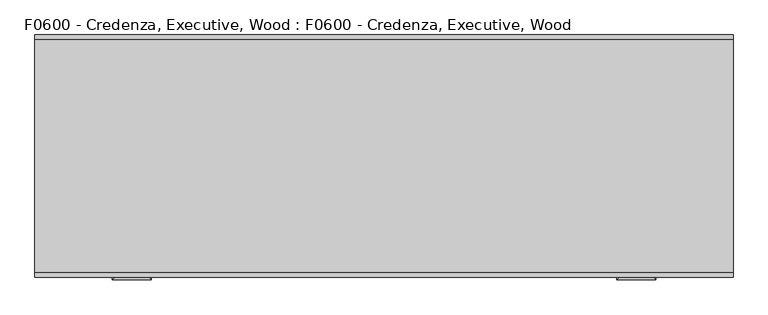
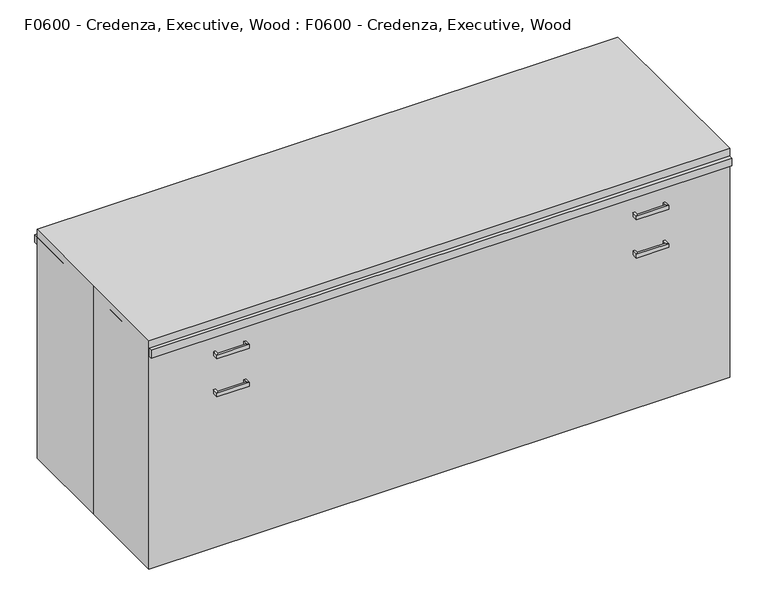
"""IFC4 building model written with IfcOpenShell, lengths in millimetres: proxy geometry, F0600 - Credenza, Executive, Wood : F0600 - Credenza, Executive, Wood."""

import ifcopenshell
import ifcopenshell.guid

model = None  # the IFC model being written
_history = None  # IfcOwnerHistory: only IFC2X3 demands one
_inside = {}  # id of a spatial element -> (the spatial element, [elements in it])
_under = {}  # id of a project, library or spatial element -> (it, [spatial elements below it])
_declared = {}  # id of a project -> (the project, [libraries it declares])
_typed = {}  # id of a type object -> (the type object, [elements of that type])
_made_of = {}  # id of a material, layer set ... -> (it, [elements and type objects made of it])


def new_model(schema):
    """Start an empty IFC model of exactly this schema.

    Asked for "IFC4X3", IfcOpenShell would pick the latest addendum, in which some entities
    have other attributes; the version numbers below select the first issue.
    IFC2X3 requires an IfcOwnerHistory on every rooted entity: one is made here for all.
    """
    global model, _history
    if schema == "IFC4X3":
        model = ifcopenshell.file(schema_version=(4, 3, 0, 0))
    else:
        model = ifcopenshell.file(schema=schema)
    _inside.clear()
    _under.clear()
    _declared.clear()
    _typed.clear()
    _made_of.clear()
    _history = None
    if model.schema == "IFC2X3":
        org = make("IfcOrganization", Name="unknown")
        user = make(
            "IfcPersonAndOrganization",
            ThePerson=make("IfcPerson", FamilyName="unknown"),
            TheOrganization=org,
        )
        app = make(
            "IfcApplication",
            ApplicationDeveloper=org,
            Version="unknown",
            ApplicationFullName="unknown",
            ApplicationIdentifier="unknown",
        )
        _history = make(
            "IfcOwnerHistory",
            OwningUser=user,
            OwningApplication=app,
            ChangeAction="ADDED",
            CreationDate=0,
        )
    return model


def make(cls, **values):
    """One entity of the class cls with the attributes given. An attribute that is None is left unset."""
    return model.create_entity(
        cls, **{name: value for name, value in values.items() if value is not None}
    )


def rooted(cls, **values):
    """An entity with a GlobalId (a new one), such as an element, a storey or a relation."""
    return make(cls, GlobalId=ifcopenshell.guid.new(), OwnerHistory=_history, **values)


def si_unit(unit_type, name, prefix=None):
    """IfcSIUnit, for example si_unit("LENGTHUNIT", "METRE", prefix="MILLI")."""
    return make("IfcSIUnit", UnitType=unit_type, Prefix=prefix, Name=name)


def assignment(units):
    """IfcUnitAssignment: the units of a project."""
    return None if units is None else make("IfcUnitAssignment", Units=units)


def point(xyz):
    """IfcCartesianPoint."""
    return None if xyz is None else make("IfcCartesianPoint", Coordinates=xyz)


def direction(xyz):
    """IfcDirection."""
    return None if xyz is None else make("IfcDirection", DirectionRatios=xyz)


def frame(location, z_axis=None, x_axis=None):
    """IfcAxis2Placement3D, a coordinate frame: its origin and axes. An axis left out is left unset."""
    return make(
        "IfcAxis2Placement3D",
        Location=point(location),
        Axis=direction(z_axis),
        RefDirection=direction(x_axis),
    )


def origin():
    """The frame at (0, 0, 0) with its axes left unset."""
    return frame((0.0, 0.0, 0.0))


def origin_with_axes():
    """The frame at (0, 0, 0) with the z axis (0, 0, 1) and the x axis (1, 0, 0) written out."""
    return frame((0.0, 0.0, 0.0), z_axis=(0.0, 0.0, 1.0), x_axis=(1.0, 0.0, 0.0))


def place(relative_to, where):
    """IfcLocalPlacement: puts the frame where relative to a parent placement (None: the world)."""
    return make(
        "IfcLocalPlacement", PlacementRelTo=relative_to, RelativePlacement=where
    )


def context(
    kind, dimensions, precision=None, world=None, true_north=None, identifier=None
):
    """IfcGeometricRepresentationContext, for example the 3D "Model" context."""
    return make(
        "IfcGeometricRepresentationContext",
        ContextIdentifier=identifier,
        ContextType=kind,
        CoordinateSpaceDimension=dimensions,
        Precision=precision,
        WorldCoordinateSystem=world,
        TrueNorth=true_north,
    )


def project(units=None, contexts=None):
    """IfcProject with its units and contexts."""
    return rooted(
        "IfcProject",
        Name="project",
        RepresentationContexts=contexts,
        UnitsInContext=assignment(units),
    )


def spatial(cls, under=None, at=None, **own):
    """A site, building, storey or space (cls), placed at a placement, below another one or the project."""
    s = rooted(cls, ObjectPlacement=at, **own)
    if under is not None:
        _under.setdefault(under.id(), (under, []))[1].append(s)
    return s


def polyline(points):
    """IfcPolyline through the points."""
    return make("IfcPolyline", Points=[point(p) for p in points])


def outline(outer, holes=None, kind="AREA"):
    """IfcArbitraryClosedProfileDef: a profile drawn as a closed curve; with holes, ...WithVoids."""
    if holes is None:
        return make("IfcArbitraryClosedProfileDef", ProfileType=kind, OuterCurve=outer)
    return make(
        "IfcArbitraryProfileDefWithVoids",
        ProfileType=kind,
        OuterCurve=outer,
        InnerCurves=holes,
    )


def extrude(swept, where, along, depth):
    """IfcExtrudedAreaSolid: the profile swept, set in the frame where, extruded along a direction by depth."""
    return make(
        "IfcExtrudedAreaSolid",
        SweptArea=swept,
        Position=where,
        ExtrudedDirection=direction(along),
        Depth=depth,
    )


def faces_of(points, faces, orient=None, outer=None):
    """IfcFace entities. A face is a list of loops; a loop is a list of indices into points, from 0.

    orient and outer hold one flag for each loop. By default every Orientation is true, the
    first loop of a face is its IfcFaceOuterBound and the others are IfcFaceBound.
    """
    made = []
    for i, loops in enumerate(faces):
        bounds = []
        for j, loop in enumerate(loops):
            is_outer = j == 0 if outer is None else outer[i][j]
            bounds.append(
                make(
                    "IfcFaceOuterBound" if is_outer else "IfcFaceBound",
                    Bound=make("IfcPolyLoop", Polygon=[points[k] for k in loop]),
                    Orientation=True if orient is None else orient[i][j],
                )
            )
        made.append(make("IfcFace", Bounds=bounds))
    return made


def faceted_brep(points, faces, orient=None, outer=None, voids=None):
    """IfcFacetedBrep: a solid bounded by flat faces; with voids (closed shells), ...WithVoids."""
    shared = [point(p) for p in points]
    hull = make("IfcClosedShell", CfsFaces=faces_of(shared, faces, orient, outer))
    if voids is None:
        return make("IfcFacetedBrep", Outer=hull)
    return make(
        "IfcFacetedBrepWithVoids",
        Outer=hull,
        Voids=[
            make(cls, CfsFaces=faces_of(shared, fs, o, b)) for cls, fs, o, b in voids
        ],
    )


def shape(context_of_items, identifier, shape_type, items):
    """IfcShapeRepresentation: the items that make up one representation, for example the "Body"."""
    return make(
        "IfcShapeRepresentation",
        ContextOfItems=context_of_items,
        RepresentationIdentifier=identifier,
        RepresentationType=shape_type,
        Items=items,
    )


def source(mapping_origin, context_of_items, identifier, shape_type, items):
    """IfcRepresentationMap: a shape defined once, which mapped items show again and again."""
    return make(
        "IfcRepresentationMap",
        MappingOrigin=mapping_origin,
        MappedRepresentation=shape(context_of_items, identifier, shape_type, items),
    )


def transform(
    local_origin,
    x_axis=None,
    y_axis=None,
    z_axis=None,
    scale=None,
    scale2=None,
    scale3=None,
    uniform=True,
):
    """IfcCartesianTransformationOperator3D, or its non-uniform kind. x_axis, y_axis, z_axis: its Axis1, 2, 3."""
    if uniform:
        return make(
            "IfcCartesianTransformationOperator3D",
            Axis1=direction(x_axis),
            Axis2=direction(y_axis),
            LocalOrigin=point(local_origin),
            Scale=scale,
            Axis3=direction(z_axis),
        )
    return make(
        "IfcCartesianTransformationOperator3DnonUniform",
        Axis1=direction(x_axis),
        Axis2=direction(y_axis),
        LocalOrigin=point(local_origin),
        Scale=scale,
        Axis3=direction(z_axis),
        Scale2=scale2,
        Scale3=scale3,
    )


def mapped(mapping_source, mapping_target):
    """IfcMappedItem: shows the shape of a source again, moved by a transform."""
    return make(
        "IfcMappedItem", MappingSource=mapping_source, MappingTarget=mapping_target
    )


def made_of(thing, what):
    """Note that an element or type object is made of a material, layer set ...; save() writes the relation."""
    if what is not None:
        _made_of.setdefault(what.id(), (what, []))[1].append(thing)
    return thing


def element(
    cls,
    number,
    at=None,
    inside=None,
    cuts=None,
    type_object=None,
    material=None,
    context=None,
    identifier="Body",
    shape_type=None,
    held_by="IfcProductDefinitionShape",
    body=None,
    shapes=None,
    **own,
):
    """One element of the class cls, such as IfcWall. Its Tag is "e" and its number.

    at: its placement. inside: the storey or other place that contains it. cuts: it is an
    opening in that element (IfcRelVoidsElement). A single representation is given by context,
    identifier, shape_type and body (its items); several are given by shapes. held_by: the class
    of the entity that holds the representations. save() writes the other relations.
    """
    e = rooted(cls, Tag="e%d" % number, ObjectPlacement=at, **own)
    if body is not None:
        shapes = [shape(context, identifier, shape_type, body)]
    if shapes is not None:
        e.Representation = make(held_by, Representations=shapes)
    if inside is not None:
        _inside.setdefault(inside.id(), (inside, []))[1].append(e)
    if cuts is not None:
        rooted(
            "IfcRelVoidsElement", RelatingBuildingElement=cuts, RelatedOpeningElement=e
        )
    if type_object is not None:
        _typed.setdefault(type_object.id(), (type_object, []))[1].append(e)
    return made_of(e, material)


def aggregate(whole, parts):
    """IfcRelAggregates: a whole, such as a stair, and the parts it consists of."""
    return rooted("IfcRelAggregates", RelatingObject=whole, RelatedObjects=parts)


def save(model, path):
    """Write the relations noted so far, then the file.

    IfcRelAggregates (storeys below a building ...), IfcRelContainedInSpatialStructure (elements
    in a storey), IfcRelDefinesByType, IfcRelAssociatesMaterial and IfcRelDeclares: one each for
    every whole, place, type object, material and project.
    """
    for whole, parts in _under.values():
        aggregate(whole, parts)
    for where, things in _inside.values():
        rooted(
            "IfcRelContainedInSpatialStructure",
            RelatedElements=things,
            RelatingStructure=where,
        )
    for kind, things in _typed.values():
        rooted("IfcRelDefinesByType", RelatedObjects=things, RelatingType=kind)
    for what, things in _made_of.values():
        rooted("IfcRelAssociatesMaterial", RelatedObjects=things, RelatingMaterial=what)
    for by, libraries in _declared.values():
        rooted("IfcRelDeclares", RelatingContext=by, RelatedDefinitions=libraries)
    model.write(path)


def f0600_credenza_executive_wood_f0600_credenza_executive_wood_160093f6(model_context):
    return source(origin(), model_context, "Body", "SolidModel", [
        faceted_brep([(-704.85, -298.45, 527.05), (-704.85, -298.45, 514.35), (-711.2, -298.45, 514.35), (-711.2, -298.45, 527.05), (-704.85, -317.5, 527.05), (-704.85, -317.5, 514.35), (-711.2, -323.85, 514.35), (-711.2, -323.85, 527.05), (-615.95, -317.5, 527.05), (-615.95, -317.5, 514.35), (-609.6, -323.85, 514.35), (-609.6, -323.85, 527.05), (-615.95, -298.45, 527.05), (-609.6, -298.45, 527.05), (-609.6, -298.45, 514.35), (-615.95, -298.45, 514.35)], [[[0, 1, 2, 3]], [[1, 0, 4, 5]], [[2, 1, 5, 6]], [[3, 2, 6, 7]], [[0, 3, 7, 4]], [[5, 4, 8, 9]], [[6, 5, 9, 10]], [[7, 6, 10, 11]], [[4, 7, 11, 8]], [[12, 13, 14, 15]], [[9, 8, 12, 15]], [[10, 9, 15, 14]], [[11, 10, 14, 13]], [[8, 11, 13, 12]]]),
        faceted_brep([(-704.85, -298.45, 654.05), (-704.85, -298.45, 641.35), (-711.2, -298.45, 641.35), (-711.2, -298.45, 654.05), (-704.85, -317.5, 654.05), (-704.85, -317.5, 641.35), (-711.2, -323.85, 641.35), (-711.2, -323.85, 654.05), (-615.95, -317.5, 654.05), (-615.95, -317.5, 641.35), (-609.6, -323.85, 641.35), (-609.6, -323.85, 654.05), (-615.95, -298.45, 654.05), (-609.6, -298.45, 654.05), (-609.6, -298.45, 641.35), (-615.95, -298.45, 641.35)], [[[0, 1, 2, 3]], [[1, 0, 4, 5]], [[2, 1, 5, 6]], [[3, 2, 6, 7]], [[0, 3, 7, 4]], [[5, 4, 8, 9]], [[6, 5, 9, 10]], [[7, 6, 10, 11]], [[4, 7, 11, 8]], [[12, 13, 14, 15]], [[9, 8, 12, 15]], [[10, 9, 15, 14]], [[11, 10, 14, 13]], [[8, 11, 13, 12]]]),
        faceted_brep([(615.95, -298.45, 654.1373112), (615.95, -298.45, 641.4373112), (609.6, -298.45, 641.4373112), (609.6, -298.45, 654.1373112), (615.95, -317.5, 654.1373112), (615.95, -317.5, 641.4373112), (609.6, -323.85, 641.4373112), (609.6, -323.85, 654.1373112), (704.85, -317.5, 654.1373112), (704.85, -317.5, 641.4373112), (711.2, -323.85, 641.4373112), (711.2, -323.85, 654.1373112), (704.85, -298.45, 654.1373112), (711.2, -298.45, 654.1373112), (711.2, -298.45, 641.4373112), (704.85, -298.45, 641.4373112)], [[[0, 1, 2, 3]], [[1, 0, 4, 5]], [[2, 1, 5, 6]], [[3, 2, 6, 7]], [[0, 3, 7, 4]], [[5, 4, 8, 9]], [[6, 5, 9, 10]], [[7, 6, 10, 11]], [[4, 7, 11, 8]], [[12, 13, 14, 15]], [[9, 8, 12, 15]], [[10, 9, 15, 14]], [[11, 10, 14, 13]], [[8, 11, 13, 12]]]),
        faceted_brep([(615.95, -298.45, 527.05), (615.95, -298.45, 514.35), (609.6, -298.45, 514.35), (609.6, -298.45, 527.05), (615.95, -317.5, 527.05), (615.95, -317.5, 514.35), (609.6, -323.85, 514.35), (609.6, -323.85, 527.05), (704.85, -317.5, 527.05), (704.85, -317.5, 514.35), (711.2, -323.85, 514.35), (711.2, -323.85, 527.05), (704.85, -298.45, 527.05), (711.2, -298.45, 527.05), (711.2, -298.45, 514.35), (704.85, -298.45, 514.35)], [[[0, 1, 2, 3]], [[1, 0, 4, 5]], [[2, 1, 5, 6]], [[3, 2, 6, 7]], [[0, 3, 7, 4]], [[5, 4, 8, 9]], [[6, 5, 9, 10]], [[7, 6, 10, 11]], [[4, 7, 11, 8]], [[12, 13, 14, 15]], [[9, 8, 12, 15]], [[10, 9, 15, 14]], [[11, 10, 14, 13]], [[8, 11, 13, 12]]]),
        extrude(outline(polyline([(-914.4, 304.8), (914.4, 304.8), (914.4, -304.8), (-914.4, -304.8), (-914.4, 0.0), (-914.4, 304.8)])), origin_with_axes(), (0.0, 0.0, 1.0), 762.0),
        faceted_brep([(889.0, 317.5, 711.2), (-889.0, 317.5, 711.2), (-889.0, -292.1, 711.2), (889.0, -292.1, 711.2), (889.0, 317.5, 152.4), (889.0, -292.1, 152.4), (-889.0, -292.1, 152.4), (-889.0, 317.5, 152.4), (-431.8, -292.1, 692.15), (431.8, -292.1, 692.15), (431.8, -292.1, 171.45), (-431.8, -292.1, 171.45), (431.8, 298.45, 692.15), (-431.8, 298.45, 692.15), (-431.8, 298.45, 171.45), (431.8, 298.45, 171.45)], [[[0, 1, 2, 3]], [[4, 5, 6, 7]], [[1, 0, 4, 7]], [[2, 1, 7, 6]], [[3, 2, 6, 5], [8, 9, 10, 11]], [[0, 3, 5, 4]], [[12, 13, 14, 15]], [[13, 12, 9, 8]], [[14, 13, 8, 11]], [[15, 14, 11, 10]], [[12, 15, 10, 9]]]),
        extrude(outline(polyline([(431.8, -259.1517862), (-19.05, -259.1517862), (-19.05, -246.4517862), (431.8, -246.4517862), (431.8, -259.1517862)])), frame((0.0, 0.0, 171.45), z_axis=(0.0, 0.0, 1.0), x_axis=(1.0, 0.0, 0.0)), (0.0, 0.0, 1.0), 520.7),
        extrude(outline(polyline([(20.4311852, -271.8517862), (-431.8, -271.8517862), (-431.8, -259.1517862), (20.4311852, -259.1517862), (20.4311852, -271.8517862)])), frame((0.0, 0.0, 171.45), z_axis=(0.0, 0.0, 1.0), x_axis=(1.0, 0.0, 0.0)), (0.0, 0.0, 1.0), 520.7),
        faceted_brep([(787.4, 317.5, 152.4), (787.4, 215.9, 152.4), (889.0, 215.9, 152.4), (889.0, 317.5, 152.4), (812.8, 317.5, 0.0), (889.0, 317.5, 0.0), (889.0, 241.3, 0.0), (812.8, 241.3, 0.0)], [[[0, 1, 2, 3]], [[4, 5, 6, 7]], [[4, 7, 1, 0]], [[7, 6, 2, 1]], [[6, 5, 3, 2]], [[5, 4, 0, 3]]]),
        extrude(outline(polyline([(869.95, -298.45), (431.8, -298.45), (431.8, -292.1), (869.95, -292.1), (869.95, -298.45)])), frame((0.0, 0.0, 584.2), z_axis=(0.0, 0.0, 1.0), x_axis=(1.0, 0.0, 0.0)), (0.0, 0.0, 1.0), 107.95),
        extrude(outline(polyline([(869.95, -298.45), (431.8, -298.45), (431.8, -292.1), (869.95, -292.1), (869.95, -298.45)])), frame((0.0, 0.0, 171.45), z_axis=(0.0, 0.0, 1.0), x_axis=(1.0, 0.0, 0.0)), (0.0, 0.0, 1.0), 393.7),
        extrude(outline(polyline([(-431.8, -298.45), (-869.95, -298.45), (-869.95, -292.1), (-431.8, -292.1), (-431.8, -298.45)])), frame((0.0, 0.0, 584.2), z_axis=(0.0, 0.0, 1.0), x_axis=(1.0, 0.0, 0.0)), (0.0, 0.0, 1.0), 107.95),
        extrude(outline(polyline([(-431.8, -298.45), (-869.95, -298.45), (-869.95, -292.1), (-431.8, -292.1), (-431.8, -298.45)])), frame((0.0, 0.0, 171.45), z_axis=(0.0, 0.0, 1.0), x_axis=(1.0, 0.0, 0.0)), (0.0, 0.0, 1.0), 393.7),
        faceted_brep([(-787.4, -292.1, 152.4), (-787.4, -190.5, 152.4), (-889.0, -190.5, 152.4), (-889.0, -292.1, 152.4), (-812.8, -292.1, 0.0), (-889.0, -292.1, 0.0), (-889.0, -215.9, 0.0), (-812.8, -215.9, 0.0)], [[[0, 1, 2, 3]], [[4, 5, 6, 7]], [[4, 7, 1, 0]], [[7, 6, 2, 1]], [[6, 5, 3, 2]], [[5, 4, 0, 3]]]),
        faceted_brep([(-787.4, 317.5, 152.4), (-889.0, 317.5, 152.4), (-889.0, 215.9, 152.4), (-787.4, 215.9, 152.4), (-812.8, 317.5, 0.0), (-812.8, 241.3, 0.0), (-889.0, 241.3, 0.0), (-889.0, 317.5, 0.0)], [[[0, 1, 2, 3]], [[4, 5, 6, 7]], [[4, 7, 1, 0]], [[7, 6, 2, 1]], [[6, 5, 3, 2]], [[5, 4, 0, 3]]]),
        faceted_brep([(787.4, -292.1, 152.4), (889.0, -292.1, 152.4), (889.0, -190.5, 152.4), (787.4, -190.5, 152.4), (812.8, -292.1, 0.0), (812.8, -215.9, 0.0), (889.0, -215.9, 0.0), (889.0, -292.1, 0.0)], [[[0, 1, 2, 3]], [[4, 5, 6, 7]], [[4, 7, 1, 0]], [[7, 6, 2, 1]], [[6, 5, 3, 2]], [[5, 4, 0, 3]]]),
        extrude(outline(polyline([(914.4, 317.5), (914.4, -317.5), (-914.4, -317.5), (-914.4, 317.5), (914.4, 317.5)])), frame((0.0, 0.0, 711.2), z_axis=(0.0, 0.0, 1.0), x_axis=(1.0, 0.0, 0.0)), (0.0, 0.0, 1.0), 25.4),
    ])


if __name__ == "__main__":
    model = new_model("IFC4")
    model_context = context("Model", 3, world=origin())
    ifc_project = project(units=[si_unit("LENGTHUNIT", "METRE", prefix="MILLI")], contexts=[model_context])
    site = spatial("IfcSite", under=ifc_project)
    building = spatial("IfcBuilding", under=site)
    placement = place(None, origin())
    f0600_credenza_executive_wood_f0600_credenza_executive_wood_shape = f0600_credenza_executive_wood_f0600_credenza_executive_wood_160093f6(model_context)
    element("IfcBuildingElementProxy", 1, Name="F0600 - Credenza, Executive, Wood : F0600 - Credenza, Executive, Wood", ObjectType="F0600 - Credenza, Executive, Wood : F0600 - Credenza, Executive, Wood", at=placement, inside=building, context=model_context, shape_type="MappedRepresentation", body=[
        mapped(f0600_credenza_executive_wood_f0600_credenza_executive_wood_shape, transform((0.0, 0.0, 0.0), x_axis=(1.0, 0.0, 0.0), y_axis=(0.0, 1.0, 0.0), z_axis=(0.0, 0.0, 1.0))),
    ])
    save(model, "model.ifc")

# Revit data of these elements
# Project information
#   Sheets - Total = "6"
#   Project Issue Date = "Issue Date"
#   Project Status = "Project Status"
#   Client Name = "Owner"
#   Project Address = "Enter address here"
#   Project Name = "Project Name"
#   Project Number = "Project Number"
#   Publication Date = "30-Jan-15"
# Type "F0600 - Credenza, Executive, Wood : F0600 - Credenza, Executive, Wood"
#   Watts2 = "0"
#   Watts1 = "0"
#   Unit_Issue = "EA"
#   UTIL_6_Misc = "-"
#   UTIL_5_NonMedGas = "-"
#   UTIL_4_MiscGas = "-"
#   UTIL_3_MedGas = "-"
#   UTIL_2_Elec = "-"
#   UTIL_1_WaterDrain = "-"
#   Nomenclature = "Credenza, Executive, Wood"
#   NSN = "7110"
#   Location [instance default] = ""
#   JSN = "F0600"
#   Fund_Source_VA = "-"
#   Fund_Source_Navy = "-"
#   Fund_Source_Army = "-"
#   Fund_Source_AF = "-"
#   ELEC_Volts2 = "0"
#   ELEC_Volts1 = "0"
#   ELEC_Phase2 = "0"
#   ELEC_Phase1 = "0"
#   ELEC_HertzSwitch = "0"
#   ELEC_HertzDependent = "0"
#   ELEC_Hertz = "0"
#   ELEC_Amps2 = "0"
#   ELEC_Amps1 = "0"
#   DetailDescription = "Executive credenza with two (2) box drawers, two (2) file drawers, a center closed storage area with adjustable shelf and floor glides."
#   CAT_VA = "C"
#   CAT_Navy = "C"
#   CAT_IHS = "-"
#   CAT_Army = "C"
#   CAT_AF = "C"
#   BTUperhour = "0"
#   Weight_IP = 332
#   DIM_Width_IP = 6' - 0"
#   DIM_Height_IP = 2' - 6"
#   DIM_Depth_IP = 2' - 0"
#   Top Material = Wood - Cherry
#   Handles/Legs Material = Metal - Chrome
#   Body Material = Laminate - Ivory, Matte
# Element 1 (IfcBuildingElementProxy, "F0600 - Credenza, Executive, Wood : F0600 - Credenza, Executive, Wood")
#   Location = "CRA02"
#   Materials on its faces: "EquipSpace"
# Materials
#   "Wood - Cherry": class "Wood", colour RGB 226 177 128, transparency 0
#   "Metal - Chrome": class "Metal", colour RGB 17 17 17, transparency 0
#   "Laminate - Ivory, Matte": class "Miscellaneous", colour RGB 247 247 239, transparency 0
#   "EquipSpace": class "Unassigned", colour RGB 221 217 195, transparency 0.5
